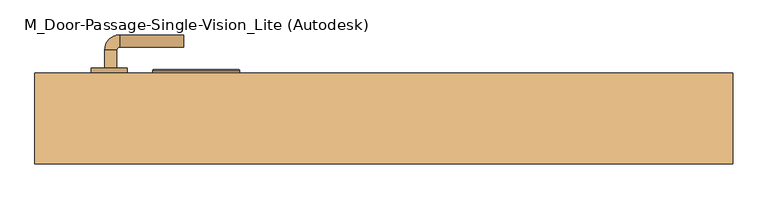
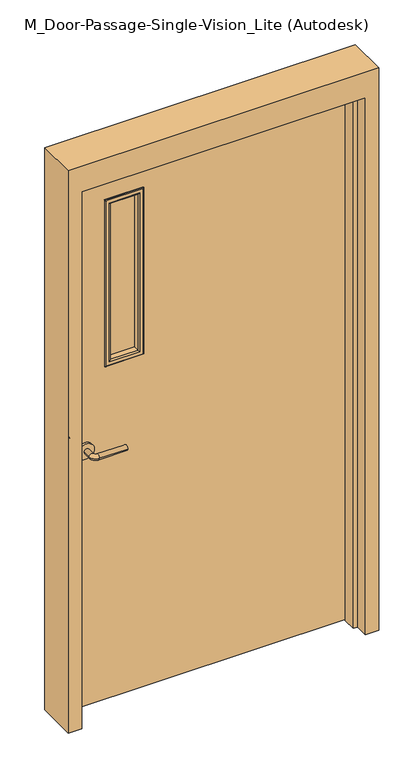
"""IFC4 building model written with IfcOpenShell, lengths in millimetres: door geometry, M_Door-Passage-Single-Vision_Lite (Autodesk) : H_DR_AMD_Single Door_Ext_Steel_1050x2100_Vision."""

from ifc_helpers import new_model, si_unit, point, frame, frame_2d, origin, place, context, project, spatial, polyline, circle_curve, ellipse_curve, trimmed, segment, composite_curve, outline, extrude, faceted_brep, source, transform, mapped, element, save
from ifc_brep_helpers import plane_surface, cylinder_surface, revolved_surface, advanced_brep


def m_door_passage_single_vision_lite_autodesk_9d2ad7b9(model_context):
    return source(origin(), model_context, "Body", "SolidModel", [
        advanced_brep(
        [(-459.990625, 123.35, 1000.0), (-439.990625, 123.35, 1000.0), (-439.990625, 93.35, 1000.0), (-459.990625, 93.35, 1000.0), (-434.990625, 88.35, 1000.0), (-434.990625, 68.35, 1000.0), (-329.990625, 68.35, 1000.0), (-329.990625, 88.35, 1000.0)],
        [
            (0, 1, circle_curve(frame((-449.990625, 123.35, 1000.0), z_axis=(0.0, 1.0, 0.0), x_axis=(1.0, 0.0, 0.0)), 10.0)),
            (1, 0, circle_curve(frame((-449.990625, 123.35, 1000.0), z_axis=(0.0, 1.0, 0.0), x_axis=(1.0, 0.0, 0.0)), 10.0)),
            (1, 2),
            (2, 3, circle_curve(frame((-449.990625, 93.35, 1000.0), z_axis=(0.0, 1.0, 0.0), x_axis=(1.0, 0.0, 0.0)), 10.0)),
            (3, 0),
            (3, 2, circle_curve(frame((-449.990625, 93.35, 1000.0), z_axis=(0.0, 1.0, 0.0), x_axis=(1.0, 0.0, 0.0)), 10.0)),
            (4, 5, circle_curve(frame((-434.990625, 78.35, 1000.0), z_axis=(-1.0, 0.0, 0.0), x_axis=(0.0, 1.0, 0.0)), 10.0)),
            (5, 3, circle_curve(frame((-434.990625, 93.35, 1000.0), z_axis=(0.0, 0.0, -1.0), x_axis=(-1.0, 0.0, 0.0)), 25.0)),
            (2, 4, circle_curve(frame((-434.990625, 93.35, 1000.0), z_axis=(0.0, 0.0, 1.0), x_axis=(-1.0, 0.0, 0.0)), 5.0)),
            (5, 4, circle_curve(frame((-434.990625, 78.35, 1000.0), z_axis=(-1.0, 0.0, 0.0), x_axis=(0.0, 1.0, 0.0)), 10.0)),
            (6, 7, circle_curve(frame((-329.990625, 78.35, 1000.0), z_axis=(1.0, 0.0, 0.0), x_axis=(0.0, 1.0, 0.0)), 10.0)),
            (7, 6, circle_curve(frame((-329.990625, 78.35, 1000.0), z_axis=(1.0, 0.0, 0.0), x_axis=(0.0, 1.0, 0.0)), 10.0)),
            (4, 7),
            (6, 5),
        ],
        [
            plane_surface(frame((-449.990625, 123.35, 1000.0), z_axis=(0.0, 1.0, 0.0), x_axis=(0.0, 0.0, 1.0))),
            cylinder_surface(frame((-449.990625, 123.35, 1000.0), z_axis=(0.0, 1.0, 0.0), x_axis=(1.0, 0.0, 0.0)), 10.0),
            revolved_surface(trimmed(ellipse_curve(frame((-449.990625, 93.35, 1000.0), z_axis=(0.0, -1.0, 0.0), x_axis=(1.0, 0.0, 0.0)), 10.0, 10.0), [point((-459.990625, 93.35, 1000.0))], [point((-439.990625, 93.35, 1000.0))], True, "CARTESIAN"), (-434.990625, 93.35, 1000.0), (0.0, 0.0, -1.0)),
            revolved_surface(trimmed(ellipse_curve(frame((-449.990625, 93.35, 1000.0), z_axis=(0.0, -1.0, 0.0), x_axis=(1.0, 0.0, 0.0)), 10.0, 10.0), [point((-439.990625, 93.35, 1000.0))], [point((-459.990625, 93.35, 1000.0))], True, "CARTESIAN"), (-434.990625, 93.35, 1000.0), (0.0, 0.0, -1.0)),
            plane_surface(frame((-329.990625, 78.35, 1000.0), z_axis=(1.0, 0.0, 0.0), x_axis=(0.0, 0.0, 1.0))),
            cylinder_surface(frame((-434.990625, 78.35, 1000.0), z_axis=(-1.0, 0.0, 0.0), x_axis=(0.0, 1.0, 0.0)), 10.0),
        ],
        [
            (0, [[1, 2]]),
            (1, [[3, 4, 5, -2]]),
            (1, [[-5, 6, -3, -1]]),
            (2, [[7, 8, -4, 9]]),
            (3, [[10, -9, -6, -8]]),
            (4, [[11, 12]]),
            (5, [[13, -11, 14, -7]]),
            (5, [[-14, -12, -13, -10]]),
        ],
    ),
        extrude(outline(composite_curve([segment(trimmed(circle_curve(frame_2d((1000.0, -452.490625)), 30.0), [point((1000.0, -482.490625))], [point((1000.0, -422.490625))], False, "CARTESIAN"), True, "CONTINUOUS"), segment(trimmed(circle_curve(frame_2d((1000.0, -452.490625)), 30.0), [point((1000.0, -422.490625))], [point((1000.0, -482.490625))], False, "CARTESIAN"), True, "CONTINUOUS")], self_intersect=False)), frame((0.0, 123.35, 0.0), z_axis=(0.0, 1.0, 0.0), x_axis=(0.0, 0.0, 1.0)), (0.0, 0.0, 1.0), 8.0),
        advanced_brep(
        [(-459.990625, 184.35, 1000.0), (-439.990625, 184.35, 1000.0), (-459.990625, 214.35, 1000.0), (-439.990625, 214.35, 1000.0), (-434.990625, 219.35, 1000.0), (-434.990625, 239.35, 1000.0), (-329.990625, 239.35, 1000.0), (-329.990625, 219.35, 1000.0)],
        [
            (0, 1, circle_curve(frame((-449.990625, 184.35, 1000.0), z_axis=(0.0, -1.0, 0.0), x_axis=(1.0, 0.0, 0.0)), 10.0)),
            (1, 0, circle_curve(frame((-449.990625, 184.35, 1000.0), z_axis=(0.0, -1.0, 0.0), x_axis=(1.0, 0.0, 0.0)), 10.0)),
            (0, 2),
            (2, 3, circle_curve(frame((-449.990625, 214.35, 1000.0), z_axis=(0.0, -1.0, 0.0), x_axis=(1.0, 0.0, 0.0)), 10.0)),
            (3, 1),
            (3, 2, circle_curve(frame((-449.990625, 214.35, 1000.0), z_axis=(0.0, -1.0, 0.0), x_axis=(1.0, 0.0, 0.0)), 10.0)),
            (4, 3, circle_curve(frame((-434.990625, 214.35, 1000.0), z_axis=(0.0, 0.0, 1.0), x_axis=(-1.0, 0.0, 0.0)), 5.0)),
            (2, 5, circle_curve(frame((-434.990625, 214.35, 1000.0), z_axis=(0.0, 0.0, -1.0), x_axis=(-1.0, 0.0, 0.0)), 25.0)),
            (5, 4, circle_curve(frame((-434.990625, 229.35, 1000.0), z_axis=(-1.0, 0.0, 0.0), x_axis=(0.0, -1.0, 0.0)), 10.0)),
            (4, 5, circle_curve(frame((-434.990625, 229.35, 1000.0), z_axis=(-1.0, 0.0, 0.0), x_axis=(0.0, -1.0, 0.0)), 10.0)),
            (6, 7, circle_curve(frame((-329.990625, 229.35, 1000.0), z_axis=(1.0, 0.0, 0.0), x_axis=(0.0, -1.0, 0.0)), 10.0)),
            (7, 6, circle_curve(frame((-329.990625, 229.35, 1000.0), z_axis=(1.0, 0.0, 0.0), x_axis=(0.0, -1.0, 0.0)), 10.0)),
            (5, 6),
            (7, 4),
        ],
        [
            plane_surface(frame((-449.990625, 184.35, 1000.0), z_axis=(0.0, -1.0, 0.0), x_axis=(0.0, 0.0, 1.0))),
            cylinder_surface(frame((-449.990625, 184.35, 1000.0), z_axis=(0.0, -1.0, 0.0), x_axis=(1.0, 0.0, 0.0)), 10.0),
            revolved_surface(trimmed(ellipse_curve(frame((-449.990625, 214.35, 1000.0), z_axis=(0.0, -1.0, 0.0), x_axis=(1.0, 0.0, 0.0)), 10.0, 10.0), [point((-459.990625, 214.35, 1000.0))], [point((-439.990625, 214.35, 1000.0))], True, "CARTESIAN"), (-434.990625, 214.35, 1000.0), (0.0, 0.0, -1.0)),
            revolved_surface(trimmed(ellipse_curve(frame((-449.990625, 214.35, 1000.0), z_axis=(0.0, -1.0, 0.0), x_axis=(1.0, 0.0, 0.0)), 10.0, 10.0), [point((-439.990625, 214.35, 1000.0))], [point((-459.990625, 214.35, 1000.0))], True, "CARTESIAN"), (-434.990625, 214.35, 1000.0), (0.0, 0.0, -1.0)),
            plane_surface(frame((-329.990625, 229.35, 1000.0), z_axis=(1.0, 0.0, 0.0), x_axis=(0.0, 0.0, 1.0))),
            cylinder_surface(frame((-434.990625, 229.35, 1000.0), z_axis=(-1.0, 0.0, 0.0), x_axis=(0.0, -1.0, 0.0)), 10.0),
        ],
        [
            (0, [[1, 2]]),
            (1, [[-1, 3, 4, 5]]),
            (1, [[-2, -5, 6, -3]]),
            (2, [[7, -4, 8, 9]]),
            (3, [[-8, -6, -7, 10]]),
            (4, [[11, 12]]),
            (5, [[-9, 13, -12, 14]]),
            (5, [[-10, -14, -11, -13]]),
        ],
    ),
        extrude(outline(composite_curve([segment(trimmed(circle_curve(frame_2d((1000.0, -452.490625)), 30.0), [point((1000.0, -482.490625))], [point((1000.0, -422.490625))], False, "CARTESIAN"), True, "CONTINUOUS"), segment(trimmed(circle_curve(frame_2d((1000.0, -452.490625)), 30.0), [point((1000.0, -422.490625))], [point((1000.0, -482.490625))], False, "CARTESIAN"), True, "CONTINUOUS")], self_intersect=False)), frame((0.0, 176.35, 0.0), z_axis=(0.0, 1.0, 0.0), x_axis=(0.0, 0.0, 1.0)), (0.0, 0.0, 1.0), 8.0),
        faceted_brep([(525.0, 126.5875, 0.0), (525.0, 176.35, 0.0), (575.0, 176.35, 0.0), (575.0, 26.35, 0.0), (525.0, 26.35, 0.0), (525.0, 75.5625, 0.0), (509.125, 75.5625, 0.0), (509.125, 126.5875, 0.0), (525.0, 126.5875, 2100.0), (525.0, 176.35, 2100.0), (-525.0, 176.35, 2100.0), (-525.0, 176.35, 0.0), (-575.0, 176.35, 0.0), (-575.0, 176.35, 2200.0), (575.0, 176.35, 2200.0), (575.0, 26.35, 2200.0), (-575.0, 26.35, 2200.0), (-575.0, 26.35, 0.0), (-525.0, 26.35, 0.0), (-525.0, 26.35, 2100.0), (525.0, 26.35, 2100.0), (525.0, 75.5625, 2100.0), (-525.0, 75.5625, 2100.0), (-525.0, 75.5625, 0.0), (-509.125, 75.5625, 0.0), (-509.125, 75.5625, 2084.125), (509.125, 75.5625, 2084.125), (509.125, 126.5875, 2084.125), (-509.125, 126.5875, 2084.125), (-509.125, 126.5875, 0.0), (-525.0, 126.5875, 0.0), (-525.0, 126.5875, 2100.0)], [[[0, 1, 2, 3, 4, 5, 6, 7]], [[1, 0, 8, 9]], [[2, 1, 9, 10, 11, 12, 13, 14]], [[3, 2, 14, 15]], [[4, 3, 15, 16, 17, 18, 19, 20]], [[5, 4, 20, 21]], [[6, 5, 21, 22, 23, 24, 25, 26]], [[7, 6, 26, 27]], [[0, 7, 27, 28, 29, 30, 31, 8]], [[9, 8, 31, 10]], [[20, 19, 22, 21]], [[26, 25, 28, 27]], [[12, 11, 30, 29, 24, 23, 18, 17]], [[11, 10, 31, 30]], [[13, 12, 17, 16]], [[19, 18, 23, 22]], [[25, 24, 29, 28]], [[15, 14, 13, 16]]]),
        extrude(outline(polyline([(2100.0, -525.0), (0.0, -525.0), (0.0, 525.0), (2100.0, 525.0), (2100.0, -525.0)]), holes=[polyline([(1947.6, -372.6), (1947.6, -245.6), (1312.6, -245.6), (1312.6, -372.6), (1947.6, -372.6)])]), frame((0.0, 131.35, 0.0), z_axis=(0.0, 1.0, 0.0), x_axis=(0.0, 0.0, 1.0)), (0.0, 0.0, 1.0), 45.0),
        extrude(outline(polyline([(-245.6, 151.35), (-372.6, 151.35), (-372.6, 156.35), (-245.6, 156.35), (-245.6, 151.35)])), frame((0.0, 0.0, 1312.6), z_axis=(0.0, 0.0, 1.0), x_axis=(1.0, 0.0, 0.0)), (0.0, 0.0, 1.0), 635.0),
        advanced_brep(
        [(-372.6, 151.35, 1312.6), (-372.6, 131.35, 1312.6), (-372.6, 131.35, 1947.6), (-372.6, 151.35, 1947.6), (-360.6, 130.35, 1324.6), (-360.6, 151.35, 1324.6), (-360.6, 151.35, 1935.6), (-360.6, 130.35, 1935.6), (-365.6, 125.35, 1319.6), (-365.6, 125.35, 1940.6), (-380.6, 127.35, 1304.6), (-378.6, 125.35, 1306.6), (-378.6, 125.35, 1953.6), (-380.6, 127.35, 1955.6), (-380.6, 131.35, 1304.6), (-380.6, 131.35, 1955.6), (-245.6, 131.35, 1947.6), (-245.6, 151.35, 1947.6), (-257.6, 151.35, 1935.6), (-257.6, 130.35, 1935.6), (-252.6, 125.35, 1940.6), (-239.6, 125.35, 1953.6), (-237.6, 127.35, 1955.6), (-237.6, 131.35, 1955.6), (-245.6, 131.35, 1312.6), (-245.6, 151.35, 1312.6), (-257.6, 151.35, 1324.6), (-257.6, 130.35, 1324.6), (-252.6, 125.35, 1319.6), (-239.6, 125.35, 1306.6), (-237.6, 127.35, 1304.6), (-237.6, 131.35, 1304.6)],
        [
            (0, 1),
            (1, 2),
            (2, 3),
            (3, 0),
            (4, 5),
            (5, 6),
            (6, 7),
            (7, 4),
            (8, 4, ellipse_curve(frame((-365.6, 130.35, 1319.6), z_axis=(-0.7071067811865475, 0.0, 0.7071067811865475), x_axis=(-0.7071067811865474, 0.0, -0.7071067811865476)), 7.0710678, 5.0)),
            (7, 9, ellipse_curve(frame((-365.6, 130.35, 1940.6), z_axis=(-0.7071067811865475, 0.0, -0.7071067811865475), x_axis=(0.7071067811865474, 0.0, -0.7071067811865476)), 7.0710678, 5.0)),
            (9, 8),
            (10, 11, ellipse_curve(frame((-378.6, 127.35, 1306.6), z_axis=(-0.7071067811865475, 0.0, 0.7071067811865475), x_axis=(-0.7071067811865474, 0.0, -0.7071067811865476)), 2.8284271, 2.0)),
            (11, 12),
            (12, 13, ellipse_curve(frame((-378.6, 127.35, 1953.6), z_axis=(-0.7071067811865475, 0.0, -0.7071067811865475), x_axis=(0.7071067811865474, 0.0, -0.7071067811865476)), 2.8284271, 2.0)),
            (13, 10),
            (14, 10),
            (13, 15),
            (15, 14),
            (2, 16),
            (16, 17),
            (17, 3),
            (6, 18),
            (18, 19),
            (19, 7),
            (19, 20, ellipse_curve(frame((-252.6, 130.35, 1940.6), z_axis=(-0.7071067811865475, 0.0, 0.7071067811865475), x_axis=(-0.7071067811865476, 0.0, -0.7071067811865474)), 7.0710678, 5.0)),
            (20, 9),
            (12, 21),
            (21, 22, ellipse_curve(frame((-239.6, 127.35, 1953.6), z_axis=(-0.7071067811865475, 0.0, 0.7071067811865475), x_axis=(-0.7071067811865476, 0.0, -0.7071067811865474)), 2.8284271, 2.0)),
            (22, 13),
            (22, 23),
            (23, 15),
            (16, 24),
            (24, 25),
            (25, 17),
            (18, 26),
            (26, 27),
            (27, 19),
            (27, 28, ellipse_curve(frame((-252.6, 130.35, 1319.6), z_axis=(0.7071067811865475, 0.0, 0.7071067811865475), x_axis=(-0.7071067811865474, 0.0, 0.7071067811865476)), 7.0710678, 5.0)),
            (28, 20),
            (21, 29),
            (29, 30, ellipse_curve(frame((-239.6, 127.35, 1306.6), z_axis=(0.7071067811865475, 0.0, 0.7071067811865475), x_axis=(-0.7071067811865474, 0.0, 0.7071067811865476)), 2.8284271, 2.0)),
            (30, 22),
            (30, 31),
            (31, 23),
            (31, 14),
            (1, 24),
            (0, 25),
            (5, 26),
            (4, 27),
            (8, 28),
            (11, 29),
            (10, 30),
        ],
        [
            plane_surface(frame((-372.6, 131.35, 1312.6), z_axis=(-1.0, 0.0, 0.0), x_axis=(0.0, 0.0, 1.0))),
            plane_surface(frame((-360.6, 151.35, 1324.6), z_axis=(1.0, 0.0, 0.0), x_axis=(0.0, 0.0, 1.0))),
            cylinder_surface(frame((-365.6, 130.35, 1312.6), z_axis=(0.0, 0.0, -1.0), x_axis=(-1.0, 0.0, 0.0)), 5.0),
            cylinder_surface(frame((-378.6, 127.35, 1312.6), z_axis=(0.0, 0.0, -1.0), x_axis=(-1.0, 0.0, 0.0)), 2.0),
            plane_surface(frame((-380.6, 127.35, 1304.6), z_axis=(-1.0, 0.0, 0.0), x_axis=(0.0, 0.0, 1.0))),
            plane_surface(frame((-372.6, 131.35, 1947.6), z_axis=(0.0, 0.0, 1.0), x_axis=(1.0, 0.0, 0.0))),
            plane_surface(frame((-360.6, 151.35, 1935.6), z_axis=(0.0, 0.0, -1.0), x_axis=(1.0, 0.0, 0.0))),
            cylinder_surface(frame((-372.6, 130.35, 1940.6), z_axis=(-1.0, 0.0, 0.0), x_axis=(0.0, 0.0, 1.0)), 5.0),
            cylinder_surface(frame((-372.6, 127.35, 1953.6), z_axis=(-1.0, 0.0, 0.0), x_axis=(0.0, 0.0, 1.0)), 2.0),
            plane_surface(frame((-380.6, 127.35, 1955.6), z_axis=(0.0, 0.0, 1.0), x_axis=(1.0, 0.0, 0.0))),
            plane_surface(frame((-245.6, 131.35, 1947.6), z_axis=(1.0, 0.0, 0.0), x_axis=(0.0, 0.0, -1.0))),
            plane_surface(frame((-257.6, 151.35, 1935.6), z_axis=(-1.0, 0.0, 0.0), x_axis=(0.0, 0.0, -1.0))),
            cylinder_surface(frame((-252.6, 130.35, 1947.6), z_axis=(0.0, 0.0, 1.0), x_axis=(1.0, 0.0, 0.0)), 5.0),
            cylinder_surface(frame((-239.6, 127.35, 1947.6), z_axis=(0.0, 0.0, 1.0), x_axis=(1.0, 0.0, 0.0)), 2.0),
            plane_surface(frame((-237.6, 127.35, 1955.6), z_axis=(1.0, 0.0, 0.0), x_axis=(0.0, 0.0, -1.0))),
            plane_surface(frame((-237.6, 131.35, 1304.6), z_axis=(0.0, 1.0, 0.0), x_axis=(-1.0, 0.0, 0.0))),
            plane_surface(frame((-245.6, 131.35, 1312.6), z_axis=(0.0, 0.0, -1.0), x_axis=(-1.0, 0.0, 0.0))),
            plane_surface(frame((-245.6, 151.35, 1312.6), z_axis=(0.0, 1.0, 0.0), x_axis=(-1.0, 0.0, 0.0))),
            plane_surface(frame((-257.6, 151.35, 1324.6), z_axis=(0.0, 0.0, 1.0), x_axis=(-1.0, 0.0, 0.0))),
            cylinder_surface(frame((-245.6, 130.35, 1319.6), z_axis=(1.0, 0.0, 0.0), x_axis=(0.0, 0.0, -1.0)), 5.0),
            plane_surface(frame((-252.6, 125.35, 1319.6), z_axis=(0.0, -1.0, 0.0), x_axis=(-1.0, 0.0, 0.0))),
            cylinder_surface(frame((-245.6, 127.35, 1306.6), z_axis=(1.0, 0.0, 0.0), x_axis=(0.0, 0.0, -1.0)), 2.0),
            plane_surface(frame((-237.6, 127.35, 1304.6), z_axis=(0.0, 0.0, -1.0), x_axis=(-1.0, 0.0, 0.0))),
        ],
        [
            (0, [[1, 2, 3, 4]]),
            (1, [[5, 6, 7, 8]]),
            (2, [[9, -8, 10, 11]]),
            (3, [[12, 13, 14, 15]]),
            (4, [[16, -15, 17, 18]]),
            (5, [[-3, 19, 20, 21]]),
            (6, [[-7, 22, 23, 24]]),
            (7, [[-10, -24, 25, 26]]),
            (8, [[-14, 27, 28, 29]]),
            (9, [[-17, -29, 30, 31]]),
            (10, [[-20, 32, 33, 34]]),
            (11, [[-23, 35, 36, 37]]),
            (12, [[-25, -37, 38, 39]]),
            (13, [[-28, 40, 41, 42]]),
            (14, [[-30, -42, 43, 44]]),
            (15, [[-31, -44, 45, -18], [46, -32, -19, -2]]),
            (16, [[-33, -46, -1, 47]]),
            (17, [[-21, -34, -47, -4], [48, -35, -22, -6]]),
            (18, [[-36, -48, -5, 49]]),
            (19, [[-38, -49, -9, 50]]),
            (20, [[51, -40, -27, -13], [-26, -39, -50, -11]]),
            (21, [[-41, -51, -12, 52]]),
            (22, [[-43, -52, -16, -45]]),
        ],
    ),
        advanced_brep(
        [(-372.6, 156.35, 1947.6), (-372.6, 176.35, 1947.6), (-372.6, 176.35, 1312.6), (-372.6, 156.35, 1312.6), (-360.6, 177.35, 1935.6), (-360.6, 156.35, 1935.6), (-360.6, 156.35, 1324.6), (-360.6, 177.35, 1324.6), (-365.6, 182.35, 1940.6), (-365.6, 182.35, 1319.6), (-380.6, 180.35, 1955.6), (-378.6, 182.35, 1953.6), (-378.6, 182.35, 1306.6), (-380.6, 180.35, 1304.6), (-380.6, 176.35, 1955.6), (-380.6, 176.35, 1304.6), (-245.6, 176.35, 1312.6), (-245.6, 156.35, 1312.6), (-257.6, 156.35, 1324.6), (-257.6, 177.35, 1324.6), (-252.6, 182.35, 1319.6), (-239.6, 182.35, 1306.6), (-237.6, 180.35, 1304.6), (-237.6, 176.35, 1304.6), (-245.6, 176.35, 1947.6), (-245.6, 156.35, 1947.6), (-257.6, 156.35, 1935.6), (-257.6, 177.35, 1935.6), (-252.6, 182.35, 1940.6), (-239.6, 182.35, 1953.6), (-237.6, 180.35, 1955.6), (-237.6, 176.35, 1955.6)],
        [
            (0, 1),
            (1, 2),
            (2, 3),
            (3, 0),
            (4, 5),
            (5, 6),
            (6, 7),
            (7, 4),
            (8, 4, ellipse_curve(frame((-365.6, 177.35, 1940.6), z_axis=(-0.7071067811865475, 0.0, -0.7071067811865475), x_axis=(-0.7071067811865474, 0.0, 0.7071067811865476)), 7.0710678, 5.0)),
            (7, 9, ellipse_curve(frame((-365.6, 177.35, 1319.6), z_axis=(-0.7071067811865475, 0.0, 0.7071067811865475), x_axis=(0.7071067811865474, 0.0, 0.7071067811865476)), 7.0710678, 5.0)),
            (9, 8),
            (10, 11, ellipse_curve(frame((-378.6, 180.35, 1953.6), z_axis=(-0.7071067811865475, 0.0, -0.7071067811865475), x_axis=(-0.7071067811865474, 0.0, 0.7071067811865476)), 2.8284271, 2.0)),
            (11, 12),
            (12, 13, ellipse_curve(frame((-378.6, 180.35, 1306.6), z_axis=(-0.7071067811865475, 0.0, 0.7071067811865475), x_axis=(0.7071067811865474, 0.0, 0.7071067811865476)), 2.8284271, 2.0)),
            (13, 10),
            (14, 10),
            (13, 15),
            (15, 14),
            (2, 16),
            (16, 17),
            (17, 3),
            (6, 18),
            (18, 19),
            (19, 7),
            (19, 20, ellipse_curve(frame((-252.6, 177.35, 1319.6), z_axis=(-0.7071067811865475, 0.0, -0.7071067811865475), x_axis=(-0.7071067811865476, 0.0, 0.7071067811865474)), 7.0710678, 5.0)),
            (20, 9),
            (12, 21),
            (21, 22, ellipse_curve(frame((-239.6, 180.35, 1306.6), z_axis=(-0.7071067811865475, 0.0, -0.7071067811865475), x_axis=(-0.7071067811865476, 0.0, 0.7071067811865474)), 2.8284271, 2.0)),
            (22, 13),
            (22, 23),
            (23, 15),
            (16, 24),
            (24, 25),
            (25, 17),
            (18, 26),
            (26, 27),
            (27, 19),
            (27, 28, ellipse_curve(frame((-252.6, 177.35, 1940.6), z_axis=(0.7071067811865475, 0.0, -0.7071067811865475), x_axis=(-0.7071067811865474, 0.0, -0.7071067811865476)), 7.0710678, 5.0)),
            (28, 20),
            (21, 29),
            (29, 30, ellipse_curve(frame((-239.6, 180.35, 1953.6), z_axis=(0.7071067811865475, 0.0, -0.7071067811865475), x_axis=(-0.7071067811865474, 0.0, -0.7071067811865476)), 2.8284271, 2.0)),
            (30, 22),
            (30, 31),
            (31, 23),
            (31, 14),
            (1, 24),
            (0, 25),
            (5, 26),
            (4, 27),
            (8, 28),
            (11, 29),
            (10, 30),
        ],
        [
            plane_surface(frame((-372.6, 176.35, 1947.6), z_axis=(-1.0, 0.0, 0.0), x_axis=(0.0, 0.0, -1.0))),
            plane_surface(frame((-360.6, 156.35, 1935.6), z_axis=(1.0, 0.0, 0.0), x_axis=(0.0, 0.0, -1.0))),
            cylinder_surface(frame((-365.6, 177.35, 1947.6), z_axis=(0.0, 0.0, 1.0), x_axis=(-1.0, 0.0, 0.0)), 5.0),
            cylinder_surface(frame((-378.6, 180.35, 1947.6), z_axis=(0.0, 0.0, 1.0), x_axis=(-1.0, 0.0, 0.0)), 2.0),
            plane_surface(frame((-380.6, 180.35, 1955.6), z_axis=(-1.0, 0.0, 0.0), x_axis=(0.0, 0.0, -1.0))),
            plane_surface(frame((-372.6, 176.35, 1312.6), z_axis=(0.0, 0.0, -1.0), x_axis=(1.0, 0.0, 0.0))),
            plane_surface(frame((-360.6, 156.35, 1324.6), z_axis=(0.0, 0.0, 1.0), x_axis=(1.0, 0.0, 0.0))),
            cylinder_surface(frame((-372.6, 177.35, 1319.6), z_axis=(-1.0, 0.0, 0.0), x_axis=(0.0, 0.0, -1.0)), 5.0),
            cylinder_surface(frame((-372.6, 180.35, 1306.6), z_axis=(-1.0, 0.0, 0.0), x_axis=(0.0, 0.0, -1.0)), 2.0),
            plane_surface(frame((-380.6, 180.35, 1304.6), z_axis=(0.0, 0.0, -1.0), x_axis=(1.0, 0.0, 0.0))),
            plane_surface(frame((-245.6, 176.35, 1312.6), z_axis=(1.0, 0.0, 0.0), x_axis=(0.0, 0.0, 1.0))),
            plane_surface(frame((-257.6, 156.35, 1324.6), z_axis=(-1.0, 0.0, 0.0), x_axis=(0.0, 0.0, 1.0))),
            cylinder_surface(frame((-252.6, 177.35, 1312.6), z_axis=(0.0, 0.0, -1.0), x_axis=(1.0, 0.0, 0.0)), 5.0),
            cylinder_surface(frame((-239.6, 180.35, 1312.6), z_axis=(0.0, 0.0, -1.0), x_axis=(1.0, 0.0, 0.0)), 2.0),
            plane_surface(frame((-237.6, 180.35, 1304.6), z_axis=(1.0, 0.0, 0.0), x_axis=(0.0, 0.0, 1.0))),
            plane_surface(frame((-237.6, 176.35, 1955.6), z_axis=(0.0, -1.0, 0.0), x_axis=(-1.0, 0.0, 0.0))),
            plane_surface(frame((-245.6, 176.35, 1947.6), z_axis=(0.0, 0.0, 1.0), x_axis=(-1.0, 0.0, 0.0))),
            plane_surface(frame((-245.6, 156.35, 1947.6), z_axis=(0.0, -1.0, 0.0), x_axis=(-1.0, 0.0, 0.0))),
            plane_surface(frame((-257.6, 156.35, 1935.6), z_axis=(0.0, 0.0, -1.0), x_axis=(-1.0, 0.0, 0.0))),
            cylinder_surface(frame((-245.6, 177.35, 1940.6), z_axis=(1.0, 0.0, 0.0), x_axis=(0.0, 0.0, 1.0)), 5.0),
            plane_surface(frame((-252.6, 182.35, 1940.6), z_axis=(0.0, 1.0, 0.0), x_axis=(-1.0, 0.0, 0.0))),
            cylinder_surface(frame((-245.6, 180.35, 1953.6), z_axis=(1.0, 0.0, 0.0), x_axis=(0.0, 0.0, 1.0)), 2.0),
            plane_surface(frame((-237.6, 180.35, 1955.6), z_axis=(0.0, 0.0, 1.0), x_axis=(-1.0, 0.0, 0.0))),
        ],
        [
            (0, [[1, 2, 3, 4]]),
            (1, [[5, 6, 7, 8]]),
            (2, [[9, -8, 10, 11]]),
            (3, [[12, 13, 14, 15]]),
            (4, [[16, -15, 17, 18]]),
            (5, [[-3, 19, 20, 21]]),
            (6, [[-7, 22, 23, 24]]),
            (7, [[-10, -24, 25, 26]]),
            (8, [[-14, 27, 28, 29]]),
            (9, [[-17, -29, 30, 31]]),
            (10, [[-20, 32, 33, 34]]),
            (11, [[-23, 35, 36, 37]]),
            (12, [[-25, -37, 38, 39]]),
            (13, [[-28, 40, 41, 42]]),
            (14, [[-30, -42, 43, 44]]),
            (15, [[-31, -44, 45, -18], [46, -32, -19, -2]]),
            (16, [[-33, -46, -1, 47]]),
            (17, [[-21, -34, -47, -4], [48, -35, -22, -6]]),
            (18, [[-36, -48, -5, 49]]),
            (19, [[-38, -49, -9, 50]]),
            (20, [[51, -40, -27, -13], [-26, -39, -50, -11]]),
            (21, [[-41, -51, -12, 52]]),
            (22, [[-43, -52, -16, -45]]),
        ],
    ),
    ])


if __name__ == "__main__":
    model = new_model("IFC4")
    model_context = context("Model", 3, world=origin())
    ifc_project = project(units=[si_unit("LENGTHUNIT", "METRE", prefix="MILLI")], contexts=[model_context])
    site = spatial("IfcSite", under=ifc_project)
    building = spatial("IfcBuilding", under=site)
    placement = place(None, origin())
    m_door_passage_single_vision_lite_autodesk_shape = m_door_passage_single_vision_lite_autodesk_9d2ad7b9(model_context)
    element("IfcDoor", 1, ObjectType="M_Door-Passage-Single-Vision_Lite (Autodesk) : H_DR_AMD_Single Door_Ext_Steel_1050x2100_Vision", at=placement, inside=building, context=model_context, shape_type="MappedRepresentation", body=[
        mapped(m_door_passage_single_vision_lite_autodesk_shape, transform((0.0, 0.0, 0.0), x_axis=(1.0, 0.0, 0.0), y_axis=(0.0, 1.0, 0.0), z_axis=(0.0, 0.0, 1.0))),
    ])
    save(model, "model.ifc")

# Revit data of these elements
# Type "M_Door-Passage-Single-Vision_Lite (Autodesk) : H_DR_AMD_Single Door_Ext_Steel_1050x2100_Vision"
#   Type Mark = "SD"
#   Assembly Code = "B2030100"
#   Analytic Construction = "Wooden"
#   Thickness = 0.0450 m
#   Thermal Resistance (R) = 0.455703 (m²·K)/W
#   Swing Angle [instance default] = 90.00°
#   Strike Height = 1.0000 m
#   Rough Width [instance default] = 1.1500 m
#   Rough Height [instance default] = 2.2000 m
#   MFOpeningHeight [instance default] = 0.1000 m
#   MFOpeningWidth [instance default] = 0.1000 m
#   Inset Calculate [instance default] = 0.1050 m
#   Masonry Inset [instance default] = 0.0250 m
#   Height = 2.1000 m
#   Width = 1.0500 m
#   Heat Transfer Coefficient (U) = 2.19465 W/(m²·K)
#   Masonry Frame Depth = 0.1500 m
#   Masonry Frame [instance default] = yes
#   Function = 1
#   Dry Wall Frame [instance default] = no
#   Panel Material = A04AQ130-BJ36_Louver_Aluminum
#   Glazing = Glass
#   Glass Stop Material = Metal - Paint Finish - Grey
#   Frame Material = Metal - Paint Finish - Grey
#   Door Handle Material = Aluminum
#   Visual Light Transmittance = 0
#   Solar Heat Gain Coefficient = 0
#   Wall Closure = (empty or 0)
# Element 1 (IfcDoor, "M_Door-Passage-Single-Vision_Lite (Autodesk) : H_DR_AMD_Single Door_Ext_Steel_1050x2100_Vision")
#   Materials on its faces: "Metal - Paint Finish - Grey", "Aluminum", "A04AQ130-BJ36_Louver_Aluminum", "Glass"
# Materials
#   "A04AQ130-BJ36_Louver_Aluminum": class "페인트", colour RGB 0 0 0, transparency 0, Cost = 0
#   "Glass": class "Glass", colour RGB 218 227 224, transparency 0.85, Description = "Soda Lime Glass", Cost = 0
#   "Metal - Paint Finish - Grey": class "Paint", colour RGB 104 104 104, transparency 0, Cost = 0
#   "Aluminum": class "Metal", colour RGB 244 244 244, transparency 0, Description = "Aluminum 6061", Cost = 0
